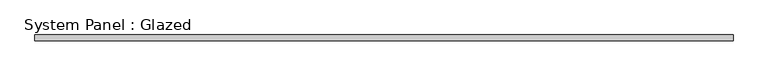
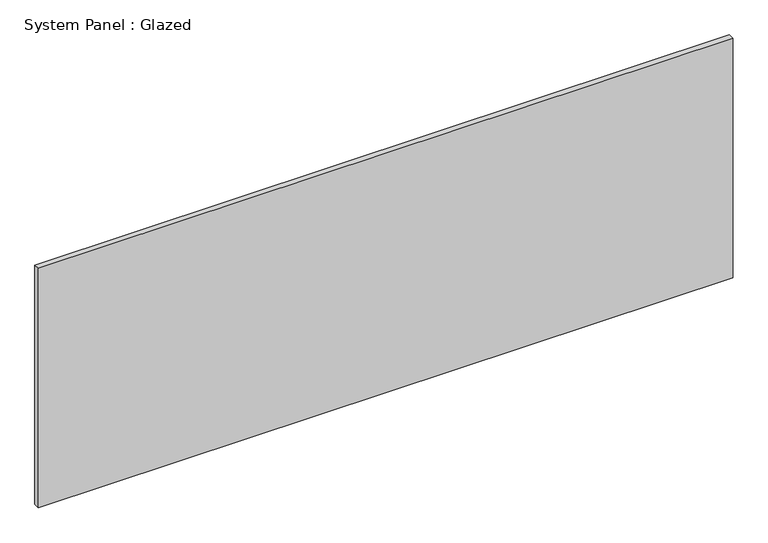
"""IFC4 building model written with IfcOpenShell, lengths in millimetres: plate geometry, System Panel : Glazed."""

import ifcopenshell
import ifcopenshell.guid

model = None  # the IFC model being written
_history = None  # IfcOwnerHistory: only IFC2X3 demands one
_inside = {}  # id of a spatial element -> (the spatial element, [elements in it])
_under = {}  # id of a project, library or spatial element -> (it, [spatial elements below it])
_declared = {}  # id of a project -> (the project, [libraries it declares])
_typed = {}  # id of a type object -> (the type object, [elements of that type])
_made_of = {}  # id of a material, layer set ... -> (it, [elements and type objects made of it])


def new_model(schema):
    """Start an empty IFC model of exactly this schema.

    Asked for "IFC4X3", IfcOpenShell would pick the latest addendum, in which some entities
    have other attributes; the version numbers below select the first issue.
    IFC2X3 requires an IfcOwnerHistory on every rooted entity: one is made here for all.
    """
    global model, _history
    if schema == "IFC4X3":
        model = ifcopenshell.file(schema_version=(4, 3, 0, 0))
    else:
        model = ifcopenshell.file(schema=schema)
    _inside.clear()
    _under.clear()
    _declared.clear()
    _typed.clear()
    _made_of.clear()
    _history = None
    if model.schema == "IFC2X3":
        org = make("IfcOrganization", Name="unknown")
        user = make(
            "IfcPersonAndOrganization",
            ThePerson=make("IfcPerson", FamilyName="unknown"),
            TheOrganization=org,
        )
        app = make(
            "IfcApplication",
            ApplicationDeveloper=org,
            Version="unknown",
            ApplicationFullName="unknown",
            ApplicationIdentifier="unknown",
        )
        _history = make(
            "IfcOwnerHistory",
            OwningUser=user,
            OwningApplication=app,
            ChangeAction="ADDED",
            CreationDate=0,
        )
    return model


def make(cls, **values):
    """One entity of the class cls with the attributes given. An attribute that is None is left unset."""
    return model.create_entity(
        cls, **{name: value for name, value in values.items() if value is not None}
    )


def rooted(cls, **values):
    """An entity with a GlobalId (a new one), such as an element, a storey or a relation."""
    return make(cls, GlobalId=ifcopenshell.guid.new(), OwnerHistory=_history, **values)


def si_unit(unit_type, name, prefix=None):
    """IfcSIUnit, for example si_unit("LENGTHUNIT", "METRE", prefix="MILLI")."""
    return make("IfcSIUnit", UnitType=unit_type, Prefix=prefix, Name=name)


def assignment(units):
    """IfcUnitAssignment: the units of a project."""
    return None if units is None else make("IfcUnitAssignment", Units=units)


def point(xyz):
    """IfcCartesianPoint."""
    return None if xyz is None else make("IfcCartesianPoint", Coordinates=xyz)


def direction(xyz):
    """IfcDirection."""
    return None if xyz is None else make("IfcDirection", DirectionRatios=xyz)


def frame(location, z_axis=None, x_axis=None):
    """IfcAxis2Placement3D, a coordinate frame: its origin and axes. An axis left out is left unset."""
    return make(
        "IfcAxis2Placement3D",
        Location=point(location),
        Axis=direction(z_axis),
        RefDirection=direction(x_axis),
    )


def origin():
    """The frame at (0, 0, 0) with its axes left unset."""
    return frame((0.0, 0.0, 0.0))


def origin_with_axes():
    """The frame at (0, 0, 0) with the z axis (0, 0, 1) and the x axis (1, 0, 0) written out."""
    return frame((0.0, 0.0, 0.0), z_axis=(0.0, 0.0, 1.0), x_axis=(1.0, 0.0, 0.0))


def place(relative_to, where):
    """IfcLocalPlacement: puts the frame where relative to a parent placement (None: the world)."""
    return make(
        "IfcLocalPlacement", PlacementRelTo=relative_to, RelativePlacement=where
    )


def context(
    kind, dimensions, precision=None, world=None, true_north=None, identifier=None
):
    """IfcGeometricRepresentationContext, for example the 3D "Model" context."""
    return make(
        "IfcGeometricRepresentationContext",
        ContextIdentifier=identifier,
        ContextType=kind,
        CoordinateSpaceDimension=dimensions,
        Precision=precision,
        WorldCoordinateSystem=world,
        TrueNorth=true_north,
    )


def project(units=None, contexts=None):
    """IfcProject with its units and contexts."""
    return rooted(
        "IfcProject",
        Name="project",
        RepresentationContexts=contexts,
        UnitsInContext=assignment(units),
    )


def spatial(cls, under=None, at=None, **own):
    """A site, building, storey or space (cls), placed at a placement, below another one or the project."""
    s = rooted(cls, ObjectPlacement=at, **own)
    if under is not None:
        _under.setdefault(under.id(), (under, []))[1].append(s)
    return s


def polyline(points):
    """IfcPolyline through the points."""
    return make("IfcPolyline", Points=[point(p) for p in points])


def outline(outer, holes=None, kind="AREA"):
    """IfcArbitraryClosedProfileDef: a profile drawn as a closed curve; with holes, ...WithVoids."""
    if holes is None:
        return make("IfcArbitraryClosedProfileDef", ProfileType=kind, OuterCurve=outer)
    return make(
        "IfcArbitraryProfileDefWithVoids",
        ProfileType=kind,
        OuterCurve=outer,
        InnerCurves=holes,
    )


def extrude(swept, where, along, depth):
    """IfcExtrudedAreaSolid: the profile swept, set in the frame where, extruded along a direction by depth."""
    return make(
        "IfcExtrudedAreaSolid",
        SweptArea=swept,
        Position=where,
        ExtrudedDirection=direction(along),
        Depth=depth,
    )


def shape(context_of_items, identifier, shape_type, items):
    """IfcShapeRepresentation: the items that make up one representation, for example the "Body"."""
    return make(
        "IfcShapeRepresentation",
        ContextOfItems=context_of_items,
        RepresentationIdentifier=identifier,
        RepresentationType=shape_type,
        Items=items,
    )


def source(mapping_origin, context_of_items, identifier, shape_type, items):
    """IfcRepresentationMap: a shape defined once, which mapped items show again and again."""
    return make(
        "IfcRepresentationMap",
        MappingOrigin=mapping_origin,
        MappedRepresentation=shape(context_of_items, identifier, shape_type, items),
    )


def transform(
    local_origin,
    x_axis=None,
    y_axis=None,
    z_axis=None,
    scale=None,
    scale2=None,
    scale3=None,
    uniform=True,
):
    """IfcCartesianTransformationOperator3D, or its non-uniform kind. x_axis, y_axis, z_axis: its Axis1, 2, 3."""
    if uniform:
        return make(
            "IfcCartesianTransformationOperator3D",
            Axis1=direction(x_axis),
            Axis2=direction(y_axis),
            LocalOrigin=point(local_origin),
            Scale=scale,
            Axis3=direction(z_axis),
        )
    return make(
        "IfcCartesianTransformationOperator3DnonUniform",
        Axis1=direction(x_axis),
        Axis2=direction(y_axis),
        LocalOrigin=point(local_origin),
        Scale=scale,
        Axis3=direction(z_axis),
        Scale2=scale2,
        Scale3=scale3,
    )


def mapped(mapping_source, mapping_target):
    """IfcMappedItem: shows the shape of a source again, moved by a transform."""
    return make(
        "IfcMappedItem", MappingSource=mapping_source, MappingTarget=mapping_target
    )


def made_of(thing, what):
    """Note that an element or type object is made of a material, layer set ...; save() writes the relation."""
    if what is not None:
        _made_of.setdefault(what.id(), (what, []))[1].append(thing)
    return thing


def element(
    cls,
    number,
    at=None,
    inside=None,
    cuts=None,
    type_object=None,
    material=None,
    context=None,
    identifier="Body",
    shape_type=None,
    held_by="IfcProductDefinitionShape",
    body=None,
    shapes=None,
    **own,
):
    """One element of the class cls, such as IfcWall. Its Tag is "e" and its number.

    at: its placement. inside: the storey or other place that contains it. cuts: it is an
    opening in that element (IfcRelVoidsElement). A single representation is given by context,
    identifier, shape_type and body (its items); several are given by shapes. held_by: the class
    of the entity that holds the representations. save() writes the other relations.
    """
    e = rooted(cls, Tag="e%d" % number, ObjectPlacement=at, **own)
    if body is not None:
        shapes = [shape(context, identifier, shape_type, body)]
    if shapes is not None:
        e.Representation = make(held_by, Representations=shapes)
    if inside is not None:
        _inside.setdefault(inside.id(), (inside, []))[1].append(e)
    if cuts is not None:
        rooted(
            "IfcRelVoidsElement", RelatingBuildingElement=cuts, RelatedOpeningElement=e
        )
    if type_object is not None:
        _typed.setdefault(type_object.id(), (type_object, []))[1].append(e)
    return made_of(e, material)


def aggregate(whole, parts):
    """IfcRelAggregates: a whole, such as a stair, and the parts it consists of."""
    return rooted("IfcRelAggregates", RelatingObject=whole, RelatedObjects=parts)


def save(model, path):
    """Write the relations noted so far, then the file.

    IfcRelAggregates (storeys below a building ...), IfcRelContainedInSpatialStructure (elements
    in a storey), IfcRelDefinesByType, IfcRelAssociatesMaterial and IfcRelDeclares: one each for
    every whole, place, type object, material and project.
    """
    for whole, parts in _under.values():
        aggregate(whole, parts)
    for where, things in _inside.values():
        rooted(
            "IfcRelContainedInSpatialStructure",
            RelatedElements=things,
            RelatingStructure=where,
        )
    for kind, things in _typed.values():
        rooted("IfcRelDefinesByType", RelatedObjects=things, RelatingType=kind)
    for what, things in _made_of.values():
        rooted("IfcRelAssociatesMaterial", RelatedObjects=things, RelatingMaterial=what)
    for by, libraries in _declared.values():
        rooted("IfcRelDeclares", RelatingContext=by, RelatedDefinitions=libraries)
    model.write(path)


def system_panel_glazed_ccd44d5c(model_context):
    return source(origin(), model_context, "Body", "SweptSolid", [
        extrude(outline(polyline([(1543.05, -44.45), (-1543.05, -44.45), (-1543.05, -19.05), (1543.05, -19.05), (1543.05, -44.45)])), origin_with_axes(), (0.0, 0.0, 1.0), 1123.95),
    ])


if __name__ == "__main__":
    model = new_model("IFC4")
    model_context = context("Model", 3, world=origin())
    ifc_project = project(units=[si_unit("LENGTHUNIT", "METRE", prefix="MILLI")], contexts=[model_context])
    site = spatial("IfcSite", under=ifc_project)
    building = spatial("IfcBuilding", under=site)
    placement = place(None, origin())
    system_panel_glazed_shape = system_panel_glazed_ccd44d5c(model_context)
    element("IfcPlate", 1, ObjectType="System Panel : Glazed", at=placement, inside=building, context=model_context, shape_type="MappedRepresentation", body=[
        mapped(system_panel_glazed_shape, transform((0.0, 0.0, 0.0), x_axis=(1.0, 0.0, 0.0), y_axis=(0.0, 1.0, 0.0), z_axis=(0.0, 0.0, 1.0))),
    ])
    save(model, "model.ifc")

# Revit data of these elements
# Type "System Panel : Glazed"
#   Construction Type Id = "GSP4R"
#   Analytic Construction = "1/8 in Pilkington single glazing"
#   Visual Light Transmittance = 0.9
#   Solar Heat Gain Coefficient = 0.86
#   Heat Transfer Coefficient (U) = 1.18115 BTU/(h·ft²·°F)
#   Define Thermal Properties by = 1
# Element 1 (IfcPlate, "System Panel : Glazed")
#   Materials on its faces: "Glass"
# Materials
#   "Glass": class "Glass", colour RGB 0 128 192, transparency 0.75, Description = "Soda Lime Glass", Cost = 0
